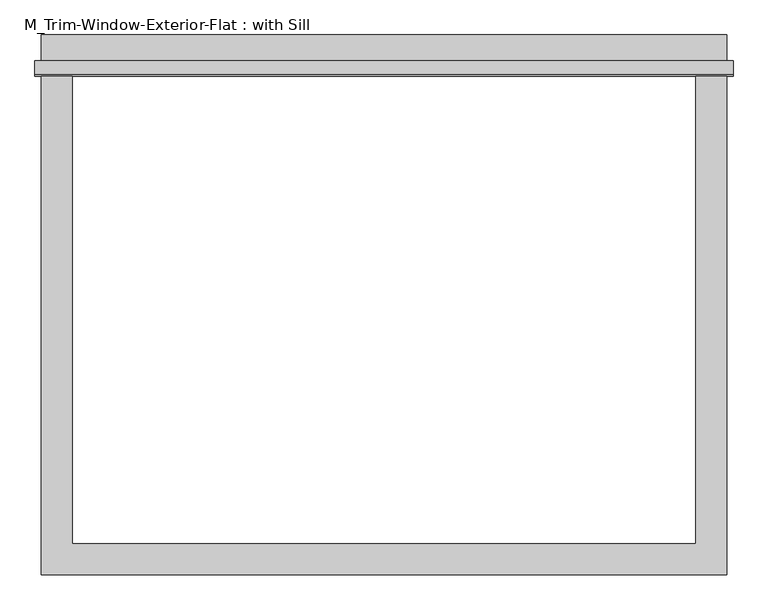
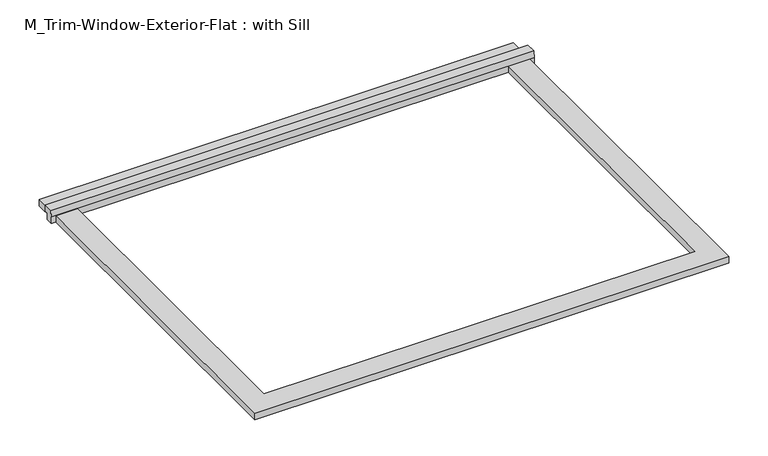
"""IFC4 building model written with IfcOpenShell, lengths in millimetres: proxy geometry, M_Trim-Window-Exterior-Flat : with Sill."""

from ifc_helpers import new_model, si_unit, frame, origin, origin_with_axes, place, context, project, spatial, polyline, outline, extrude, source, transform, mapped, element, save


def m_trim_window_exterior_flat_with_sill_46ef76a2(model_context):
    return source(origin(), model_context, "Body", "SweptSolid", [
        extrude(outline(polyline([(669.6, 934.8323709), (-669.6, 934.8323709), (-669.6, 994.8323709), (669.6, 994.8323709), (669.6, 934.8323709)])), origin_with_axes(), (0.0, 0.0, 1.0), 19.05),
        extrude(outline(polyline([(944.4, 38.1), (944.4, 19.05), (934.8323709, 19.05), (934.8323709, 0.0), (914.4, 0.0), (914.4, 19.05), (916.8580645, 38.1), (944.4, 38.1)])), frame((-682.3, 0.0, 0.0), z_axis=(1.0, 0.0, 0.0), x_axis=(0.0, 1.0, 0.0)), (0.0, 0.0, 1.0), 1364.6),
        extrude(outline(polyline([(-669.6, -60.0), (-669.6, 914.4), (-609.6, 914.4), (-609.6, 0.0), (609.6, 0.0), (609.6, 914.4), (669.6, 914.4), (669.6, -60.0), (-669.6, -60.0)])), origin_with_axes(), (0.0, 0.0, 1.0), 19.05),
    ])


if __name__ == "__main__":
    model = new_model("IFC4")
    model_context = context("Model", 3, world=origin())
    ifc_project = project(units=[si_unit("LENGTHUNIT", "METRE", prefix="MILLI")], contexts=[model_context])
    site = spatial("IfcSite", under=ifc_project)
    building = spatial("IfcBuilding", under=site)
    placement = place(None, origin())
    m_trim_window_exterior_flat_with_sill_shape = m_trim_window_exterior_flat_with_sill_46ef76a2(model_context)
    element("IfcBuildingElementProxy", 1, Name="M_Trim-Window-Exterior-Flat : with Sill", ObjectType="M_Trim-Window-Exterior-Flat : with Sill", at=placement, inside=building, context=model_context, shape_type="MappedRepresentation", body=[
        mapped(m_trim_window_exterior_flat_with_sill_shape, transform((0.0, 0.0, 0.0), x_axis=(1.0, 0.0, 0.0), y_axis=(0.0, 1.0, 0.0), z_axis=(0.0, 0.0, 1.0))),
    ])
    save(model, "model.ifc")

# Revit data of these elements
# Type "M_Trim-Window-Exterior-Flat : with Sill"
#   Trim Width = 0' - 2.3622"
#   Trim Thickness_Picture Frame = 0' - 1.1811"
#   Trim Thickness_with Sill = 0' - 0 3/4"
#   Sill Thickness = 0' - 1.1811"
#   Opening Width [instance default] = 1' - 11.62205"
#   Opening Height [instance default] = 2' - 11.43307"
#   Default Elevation = 3' - 11.24409"
#   Sill = yes
#   Picture Frame = no
#   Trim Material [instance default] = none
# Element 1 (IfcBuildingElementProxy, "M_Trim-Window-Exterior-Flat : with Sill")
#   Opening Width = 4' - 0"
#   Opening Height = 3' - 0"
#   Trim Material = Clad - White
#   Materials on its faces: "Clad - White"
# Materials
#   "Clad - White": class "Wood", colour RGB 242 242 238, transparency 0, Cost = 0
